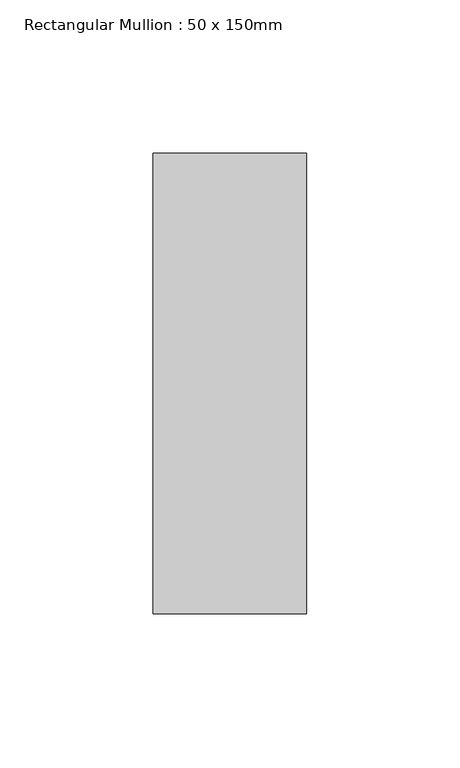
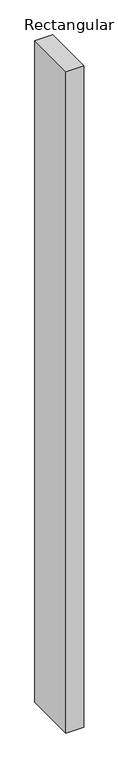
"""IFC4 building model written with IfcOpenShell, lengths in millimetres: member geometry, Rectangular Mullion : 50 x 150mm."""

from ifc_helpers import new_model, si_unit, frame, origin, place, context, project, spatial, polyline, outline, extrude, source, transform, mapped, element, save


def rectangular_mullion_50_x_150mm_2c1a111c(model_context):
    return source(origin(), model_context, "Body", "SweptSolid", [
        extrude(outline(polyline([(0.0, 75.0), (0.0, -75.0), (-50.0, -75.0), (-50.0, 75.0), (0.0, 75.0)])), frame((0.0, 0.0, -1948.3666666), z_axis=(0.0, 0.0, 1.0), x_axis=(1.0, 0.0, 0.0)), (0.0, 0.0, 1.0), 1948.3666666),
    ])


if __name__ == "__main__":
    model = new_model("IFC4")
    model_context = context("Model", 3, world=origin())
    ifc_project = project(units=[si_unit("LENGTHUNIT", "METRE", prefix="MILLI")], contexts=[model_context])
    site = spatial("IfcSite", under=ifc_project)
    building = spatial("IfcBuilding", under=site)
    placement = place(None, origin())
    rectangular_mullion_50_x_150mm_shape = rectangular_mullion_50_x_150mm_2c1a111c(model_context)
    element("IfcMember", 1, ObjectType="Rectangular Mullion : 50 x 150mm", at=placement, inside=building, context=model_context, shape_type="MappedRepresentation", body=[
        mapped(rectangular_mullion_50_x_150mm_shape, transform((0.0, 0.0, 0.0), x_axis=(1.0, 0.0, 0.0), y_axis=(0.0, 1.0, 0.0), z_axis=(0.0, 0.0, 1.0))),
    ])
    save(model, "model.ifc")

# Revit data of these elements
# Type "Rectangular Mullion : 50 x 150mm"
#   built-in parameter 1007304 = 0.492126 (stored number, unit not read)
#   built-in parameter 1007301 = 0.082021 (stored number, unit not read)
#   built-in parameter 1007300 = 0.082021 (stored number, unit not read)
# Element 1 (IfcMember, "Rectangular Mullion : 50 x 150mm")
#   Materials on its faces: "Metal - Aluminium"
# Materials
#   "Metal - Aluminium": class "Metal", colour RGB 247 247 247, transparency 0
